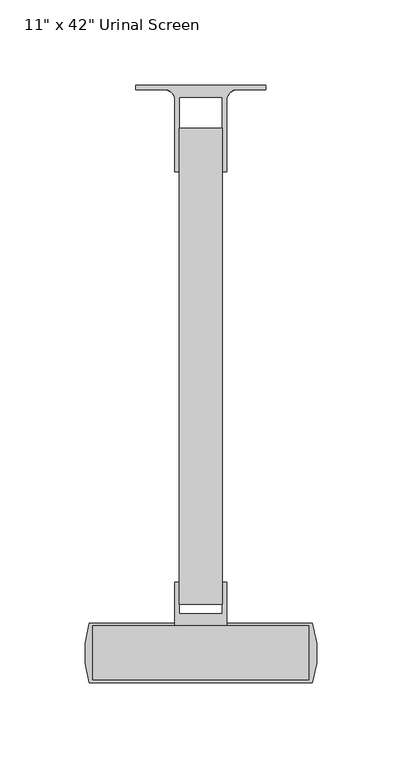
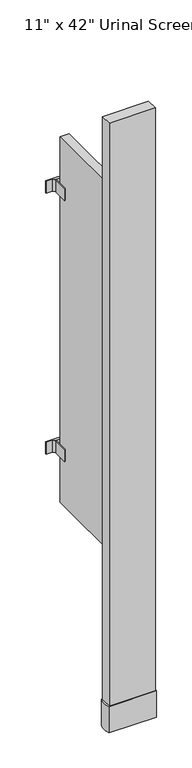
"""IFC4 building model written with IfcOpenShell, lengths in millimetres: proxy geometry."""

from ifc_helpers import new_model, si_unit, point, frame, frame_2d, origin, origin_with_axes, place, context, project, spatial, polyline, circle_curve, trimmed, segment, composite_curve, outline, extrude, source, transform, mapped, element, save


def proxy_3984ed91(model_context):
    return source(origin(), model_context, "Body", "SweptSolid", [
        extrude(outline(polyline([(-15.24, -317.5), (-15.24, -292.1), (-12.7, -292.1), (-12.7, -310.5521812), (12.7, -310.5521812), (12.7, -292.1), (15.24, -292.1), (15.24, -317.5), (-15.24, -317.5)])), frame((0.0, 0.0, 1354.1375), z_axis=(0.0, 0.0, 1.0), x_axis=(1.0, 0.0, 0.0)), (0.0, 0.0, 1.0), 25.4),
        extrude(outline(polyline([(-15.24, -317.5), (-15.24, -292.1), (-12.7, -292.1), (-12.7, -310.5521812), (12.7, -310.5521812), (12.7, -292.1), (15.24, -292.1), (15.24, -317.5), (-15.24, -317.5)])), frame((0.0, 0.0, 592.1375), z_axis=(0.0, 0.0, 1.0), x_axis=(1.0, 0.0, 0.0)), (0.0, 0.0, 1.0), 25.4),
        extrude(outline(composite_curve([segment(polyline([(38.1, 0.0), (38.1, -2.54), (21.59, -2.54)]), True, "CONTINUOUS"), segment(trimmed(circle_curve(frame_2d((21.59, -8.89)), 6.35), [point((21.59, -2.54))], [point((15.24, -8.89))], True, "CARTESIAN"), True, "CONTINUOUS"), segment(polyline([(15.24, -8.89), (15.24, -50.8), (12.7, -50.8), (12.7, -6.9478188), (-12.7, -6.9478188), (-12.7, -50.8), (-15.24, -50.8), (-15.24, -8.89)]), True, "CONTINUOUS"), segment(trimmed(circle_curve(frame_2d((-21.59, -8.89)), 6.35), [point((-15.24, -8.89))], [point((-21.59, -2.54))], True, "CARTESIAN"), True, "CONTINUOUS"), segment(polyline([(-21.59, -2.54), (-38.1, -2.54), (-38.1, 0.0), (38.1, 0.0)]), True, "CONTINUOUS")], self_intersect=False)), frame((0.0, 0.0, 1354.1375), z_axis=(0.0, 0.0, 1.0), x_axis=(1.0, 0.0, 0.0)), (0.0, 0.0, 1.0), 34.925),
        extrude(outline(composite_curve([segment(polyline([(38.1, 0.0), (38.1, -2.54), (21.59, -2.54)]), True, "CONTINUOUS"), segment(trimmed(circle_curve(frame_2d((21.59, -8.89)), 6.35), [point((21.59, -2.54))], [point((15.24, -8.89))], True, "CARTESIAN"), True, "CONTINUOUS"), segment(polyline([(15.24, -8.89), (15.24, -50.8), (12.7, -50.8), (12.7, -6.9478188), (-12.7, -6.9478188), (-12.7, -50.8), (-15.24, -50.8), (-15.24, -8.89)]), True, "CONTINUOUS"), segment(trimmed(circle_curve(frame_2d((-21.59, -8.89)), 6.35), [point((-15.24, -8.89))], [point((-21.59, -2.54))], True, "CARTESIAN"), True, "CONTINUOUS"), segment(polyline([(-21.59, -2.54), (-38.1, -2.54), (-38.1, 0.0), (38.1, 0.0)]), True, "CONTINUOUS")], self_intersect=False)), frame((0.0, 0.0, 592.1375), z_axis=(0.0, 0.0, 1.0), x_axis=(1.0, 0.0, 0.0)), (0.0, 0.0, 1.0), 34.925),
        extrude(outline(composite_curve([segment(polyline([(-65.5933846, -315.9125), (65.5933846, -315.9125)]), True, "CONTINUOUS"), segment(trimmed(circle_curve(frame_2d((9.8043529, -333.375)), 58.4581471), [point((65.5933846, -315.9125))], [point((65.5933846, -350.8375))], False, "CARTESIAN"), True, "CONTINUOUS"), segment(polyline([(65.5933846, -350.8375), (-65.5933846, -350.8375)]), True, "CONTINUOUS"), segment(trimmed(circle_curve(frame_2d((-9.8043529, -333.375)), 58.4581471), [point((-65.5933846, -350.8375))], [point((-65.5933846, -315.9125))], False, "CARTESIAN"), True, "CONTINUOUS")], self_intersect=False)), origin_with_axes(), (0.0, 0.0, 1.0), 76.2),
        extrude(outline(polyline([(-63.5, -317.5), (63.5, -317.5), (63.5, -349.25), (-63.5, -349.25), (-63.5, -317.5)])), origin_with_axes(), (0.0, 0.0, 1.0), 1778.0),
        extrude(outline(polyline([(12.7, -25.4), (12.7, -304.8), (-12.7, -304.8), (-12.7, -25.4), (12.7, -25.4)])), frame((0.0, 0.0, 457.2), z_axis=(0.0, 0.0, 1.0), x_axis=(1.0, 0.0, 0.0)), (0.0, 0.0, 1.0), 1066.8),
    ])


if __name__ == "__main__":
    model = new_model("IFC4")
    model_context = context("Model", 3, world=origin())
    ifc_project = project(units=[si_unit("LENGTHUNIT", "METRE", prefix="MILLI")], contexts=[model_context])
    site = spatial("IfcSite", under=ifc_project)
    building = spatial("IfcBuilding", under=site)
    placement = place(None, origin())
    proxy_shape = proxy_3984ed91(model_context)
    element("IfcBuildingElementProxy", 1, Name="Partition-Floor_Braced_Urinal_Screen-Bradley_Corp-St._Stl : 11\" x 42\" Urinal Screen", ObjectType="Partition-Floor_Braced_Urinal_Screen-Bradley_Corp-St._Stl : 11\" x 42\" Urinal Screen", at=placement, inside=building, context=model_context, shape_type="MappedRepresentation", body=[
        mapped(proxy_shape, transform((0.0, 0.0, 0.0), x_axis=(1.0, 0.0, 0.0), y_axis=(0.0, 1.0, 0.0), z_axis=(0.0, 0.0, 1.0))),
    ])
    save(model, "model.ifc")

# Revit data of these elements
# Type "Partition-Floor_Braced_Urinal_Screen-Bradley_Corp-St._Stl : 11\" x 42\" Urinal Screen"
#   Keynote = "M10211313.01"
#   Warranty Information = "Warranted 15 years against rust out, 5 years on chrome hardware, lifetime of the partition on the stainless steel hardware."
#   Version = "1.0"
#   URL = "http://www.bradleycorp.com"
#   Type Comments = "n/a"
#   Technical Data = "n/a"
#   OmniClass Title = "Toilet Compartment and Urinal Screens"
#   OmniClass Code = "23.25.40.14.14.11"
#   Modeling Code = "n/a"
#   Model = "Stainless Steel - Urinal Screen"
#   Material Note = "Stainless Steel Hardware Also Available - Please See www.bradleycorp.com"
#   Material = "Stainless Steel"
#   MasterFormat Title = "Toilet Compartments"
#   MasterFormat Number = "10 21 13"
#   Manufacturer = "Bradley Corporation"
#   LEED Credit = "n/a"
#   Industry Standards = "n/a"
#   Fire Rating = "n/a"
#   Description = "Restroom Partitions, Urinal Screen"
#   Copyright = "This Model Data is Property of Bradley Corporation"
#   Complies to NAFTA = "n/a"
#   Buy American Act = "To Be Determined"
#   Assembly Code = "C1010400"
#   ADA Compliant = "No"
#   Width = 0' - 11"
#   Top Stirrup Bracket Distance From Floor [instance default] = 4' - 5 5/16"
#   Top Of Pilaster = 5' - 10"
#   Percentage of Recycled Content = 0
#   Front Face Of Pilaster = 1' - 1 3/4"
#   Bottom Stirrup Bracket Distance From Floor [instance default] = 1' - 11 5/16"
#   Height = 3' - 6"
#   Distance From Floor [instance default] = 1' - 6"
#   Bracket Offset = 0' - 0 1/2"
#   Stirrup Brackets [instance default] = yes
#   Continuous Brackets [instance default] = no
#   Shoe Material = Metal - Bradley Corp - Stainless Steel Satin
#   Partition Material [instance default] = Metal - Bradley Corp - Stainless Steel Brushed
#   Hardware Material = Metal - Bradley Corp - Chrome
# Element 1 (IfcBuildingElementProxy, "Partition-Floor_Braced_Urinal_Screen-Bradley_Corp-St._Stl : 11\" x 42\" Urinal Screen")
#   Partition Material = Metal - Bradley Corp - Chrome
#   Materials on its faces: "Metal - Bradley Corp - Chrome", "Metal - Bradley Corp - Chrome Satin", "Metal - Bradley Corp - Stainless Steel Satin"
# Materials
#   "Metal - Bradley Corp - Stainless Steel Satin": class "Metal", colour RGB 189 187 185, transparency 0
#   "Metal - Bradley Corp - Stainless Steel Brushed": class "Metal", colour RGB 189 187 185, transparency 0
#   "Metal - Bradley Corp - Chrome": class "Metal", colour RGB 106 119 125, transparency 0, Cost = 0
#   "Metal - Bradley Corp - Chrome Satin": class "Metal", colour RGB 244 244 244, transparency 0
